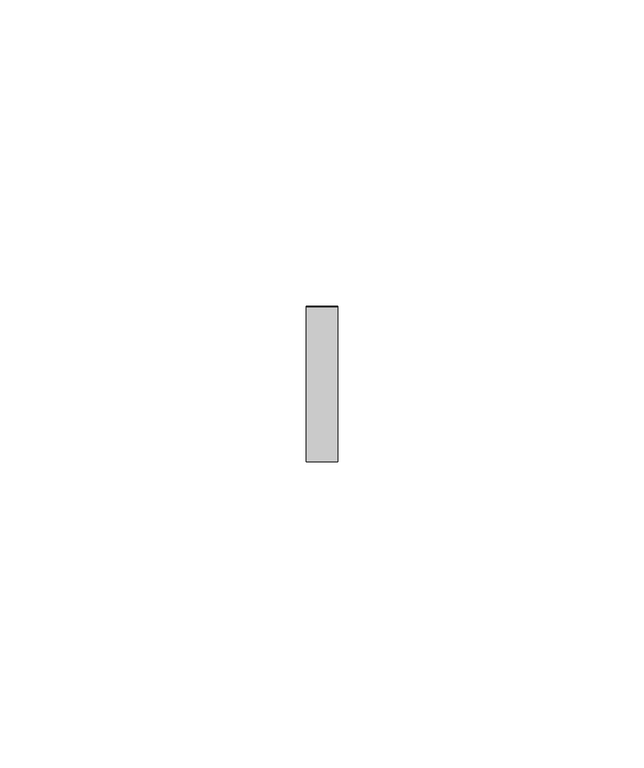
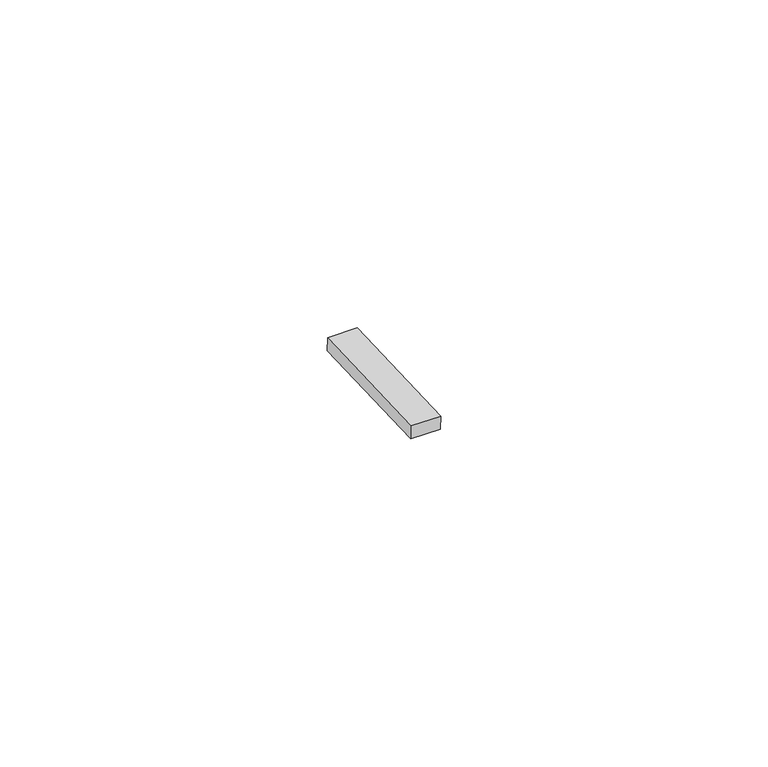
"""IFC4 building model written with IfcOpenShell, lengths in millimetres: proxy geometry, Inner panel:Inner panel:1:Inner panel:1 : Inner panel:Inner panel:300324:2:Inner panel:1:Inner panel:1 : Inner panel:Inner panel:300324:2 : Inner panel:Inner panel:1:Inner panel:1 : Inner panel:Inner panel:300324:300043:105 : Inner panel:Inner panel:1:Inner panel:1 : Inner panel:Inner panel:300324:2:Inner panel:1:Inner panel:1 : Inner panel:Inner panel:300324:2 : Inner panel:Inner panel:1:Inner panel:1 : Inner panel:Inner panel:300324:300043:308120."""

from ifc_helpers import new_model, si_unit, frame, origin, place, context, project, spatial, polyline, outline, extrude, source, transform, mapped, element, save


def generic_models_b630c318(model_context):
    return source(origin(), model_context, "Body", "SweptSolid", [
        extrude(outline(polyline([(0.0, -25.3999999), (0.0, 0.0), (5.2138089, 0.0), (5.2138089, -25.3999999), (0.0, -25.3999999)])), frame((593530.195117, -568123.7593241, 8806.3160403), z_axis=(0.0, -0.041630544712223896, 0.9991330730923502), x_axis=(-1.0, 0.0, 0.0)), (0.0, 0.0, 1.0), 2.4763745),
    ])


if __name__ == "__main__":
    model = new_model("IFC4")
    model_context = context("Model", 3, world=origin())
    ifc_project = project(units=[si_unit("LENGTHUNIT", "METRE", prefix="MILLI")], contexts=[model_context])
    site = spatial("IfcSite", under=ifc_project)
    building = spatial("IfcBuilding", under=site)
    placement = place(None, origin())
    generic_models_shape = generic_models_b630c318(model_context)
    element("IfcBuildingElementProxy", 1, Name="Inner panel:Inner panel:1:Inner panel:1 : Inner panel:Inner panel:300324:2:Inner panel:1:Inner panel:1 : Inner panel:Inner panel:300324:2 : Inner panel:Inner panel:1:Inner panel:1 : Inner panel:Inner panel:300324:300043:105 : Inner panel:Inner panel:1:Inner panel:1 : Inner panel:Inner panel:300324:2:Inner panel:1:Inner panel:1 : Inner panel:Inner panel:300324:2 : Inner panel:Inner panel:1:Inner panel:1 : Inner panel:Inner panel:300324:300043:308120", ObjectType="Inner panel:Inner panel:1:Inner panel:1 : Inner panel:Inner panel:300324:2:Inner panel:1:Inner panel:1 : Inner panel:Inner panel:300324:2 : Inner panel:Inner panel:1:Inner panel:1 : Inner panel:Inner panel:300324:300043:105 : Inner panel:Inner panel:1:Inner panel:1 : Inner panel:Inner panel:300324:2:Inner panel:1:Inner panel:1 : Inner panel:Inner panel:300324:2 : Inner panel:Inner panel:1:Inner panel:1 : Inner panel:Inner panel:300324:300043:308120", at=placement, inside=building, context=model_context, shape_type="MappedRepresentation", body=[
        mapped(generic_models_shape, transform((0.0, 0.0, 0.0), x_axis=(1.0, 0.0, 0.0), y_axis=(0.0, 1.0, 0.0), z_axis=(0.0, 0.0, 1.0))),
    ])
    save(model, "model.ifc")

# Revit data of these elements
# Type "Inner panel:Inner panel:1:Inner panel:1 : Inner panel:Inner panel:300324:2:Inner panel:1:Inner panel:1 : Inner panel:Inner panel:300324:2 : Inner panel:Inner panel:1:Inner panel:1 : Inner panel:Inner panel:300324:300043:105 : Inner panel:Inner panel:1:Inner panel:1 : Inner panel:Inner panel:300324:2:Inner panel:1:Inner panel:1 : Inner panel:Inner panel:300324:2 : Inner panel:Inner panel:1:Inner panel:1 : Inner panel:Inner panel:300324:300043:308120"
#   NameOverride = "Inner panel:Inner panel:1:Inner panel:1 : Inner panel:Inner panel:300324:2:Inner panel:1:Inner panel:1 : Inner panel:Inner panel:300324:2 : Inner panel:Inner panel:1:Inner panel:1 : Inner panel:Inner panel:300324:300043:308120"
#   ObjectTypeOverride = "Inner panel:1:Inner panel:1 : Inner panel:Inner panel:300324:2 : Inner panel:Inner panel:1:Inner panel:1 : Inner panel:Inner panel:300324:300043"
#   Reference = "Inner panel"
#   Tag = "308120"
# Element 1 (IfcBuildingElementProxy, "Inner panel:Inner panel:1:Inner panel:1 : Inner panel:Inner panel:300324:2:Inner panel:1:Inner panel:1 : Inner panel:Inner panel:300324:2 : Inner panel:Inner panel:1:Inner panel:1 : Inner panel:Inner panel:300324:300043:105 : Inner panel:Inner panel:1:Inner panel:1 : Inner panel:Inner panel:300324:2:Inner panel:1:Inner panel:1 : Inner panel:Inner panel:300324:2 : Inner panel:Inner panel:1:Inner panel:1 : Inner panel:Inner panel:300324:300043:308120")
#   Materials on its faces: "AT CLIP - 1\" WIDE NON ABSORBENT, WEATHER-RESISTANT NEOPRENE/EPDM/SBR FOAM"
# Materials
#   "AT CLIP - 1\" WIDE NON ABSORBENT, WEATHER-RESISTANT NEOPRENE/EPDM/SBR FOAM": class "Generic", colour RGB 85 85 85, transparency 0, Cost = 0
